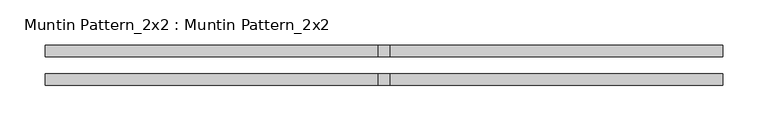
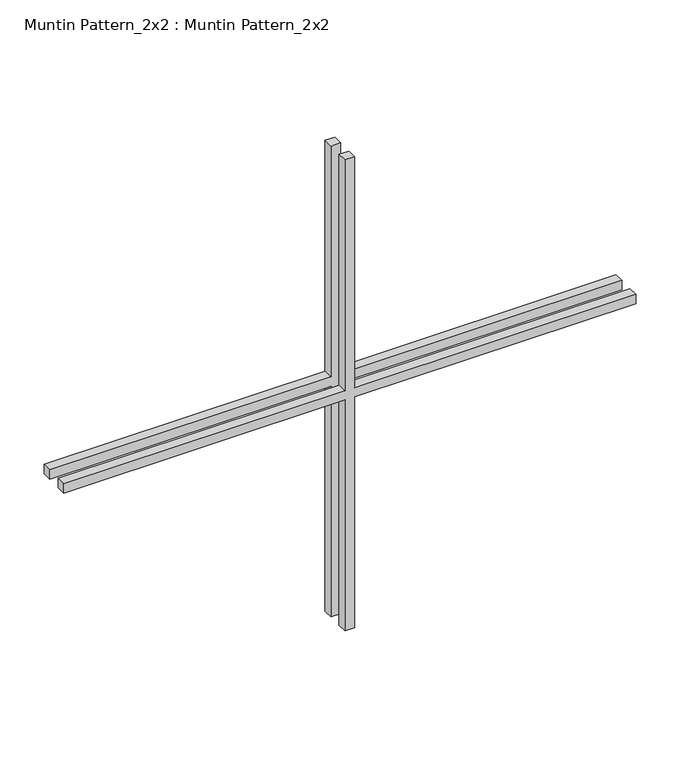
"""IFC4 building model written with IfcOpenShell, lengths in millimetres: proxy geometry, Muntin Pattern_2x2 : Muntin Pattern_2x2."""

from ifc_helpers import new_model, si_unit, frame, origin, place, context, project, spatial, polyline, outline, extrude, source, transform, mapped, element, save


def muntin_pattern_2x2_muntin_pattern_2x2_11ec8187(model_context):
    return source(origin(), model_context, "Body", "SweptSolid", [
        extrude(outline(polyline([(332.1375, -6.35), (332.1375, -374.59375), (319.4375, -374.59375), (319.4375, -6.35), (0.0, -6.35), (0.0, 6.35), (319.4375, 6.35), (319.4375, 374.59375), (332.1375, 374.59375), (332.1375, 6.35), (651.575, 6.35), (651.575, -6.35), (332.1375, -6.35)])), frame((0.0, 9.525, 0.0), z_axis=(0.0, 1.0, 0.0), x_axis=(0.0, 0.0, 1.0)), (0.0, 0.0, 1.0), 12.7),
        extrude(outline(polyline([(332.1375, -6.35), (332.1375, -374.59375), (319.4375, -374.59375), (319.4375, -6.35), (0.0, -6.35), (0.0, 6.35), (319.4375, 6.35), (319.4375, 374.59375), (332.1375, 374.59375), (332.1375, 6.35), (651.575, 6.35), (651.575, -6.35), (332.1375, -6.35)])), frame((0.0, -22.225, 0.0), z_axis=(0.0, 1.0, 0.0), x_axis=(0.0, 0.0, 1.0)), (0.0, 0.0, 1.0), 12.7),
    ])


if __name__ == "__main__":
    model = new_model("IFC4")
    model_context = context("Model", 3, world=origin())
    ifc_project = project(units=[si_unit("LENGTHUNIT", "METRE", prefix="MILLI")], contexts=[model_context])
    site = spatial("IfcSite", under=ifc_project)
    building = spatial("IfcBuilding", under=site)
    placement = place(None, origin())
    muntin_pattern_2x2_muntin_pattern_2x2_shape = muntin_pattern_2x2_muntin_pattern_2x2_11ec8187(model_context)
    element("IfcBuildingElementProxy", 1, Name="Muntin Pattern_2x2 : Muntin Pattern_2x2", ObjectType="Muntin Pattern_2x2 : Muntin Pattern_2x2", at=placement, inside=building, context=model_context, shape_type="MappedRepresentation", body=[
        mapped(muntin_pattern_2x2_muntin_pattern_2x2_shape, transform((0.0, 0.0, 0.0), x_axis=(1.0, 0.0, 0.0), y_axis=(0.0, 1.0, 0.0), z_axis=(0.0, 0.0, 1.0))),
    ])
    save(model, "model.ifc")

# Revit data of these elements
# Type "Muntin Pattern_2x2 : Muntin Pattern_2x2"
#   Width [instance default] = 121.92 cm
#   Thickness = 1.27 cm
#   Height [instance default] = 121.92 cm
#   Distance = 1.905 cm
#   Interior Material [instance default] = none
#   Exterior Material [instance default] = none
# Element 1 (IfcBuildingElementProxy, "Muntin Pattern_2x2 : Muntin Pattern_2x2")
#   Width = 74.9187 cm
#   Height = 65.1575 cm
#   Interior Material = Wood - Stained
#   Exterior Material = Clad - White
#   Materials on its faces: "Clad - White", "Wood - Stained"
# Materials
#   "Clad - White": class "Wood", colour RGB 242 242 238, transparency 0, Cost = 0
#   "Wood - Stained": class "Wood", colour RGB 224 178 126, transparency 0, Cost = 0
